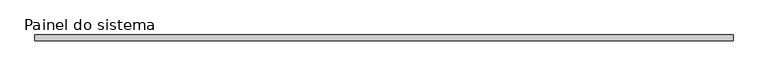
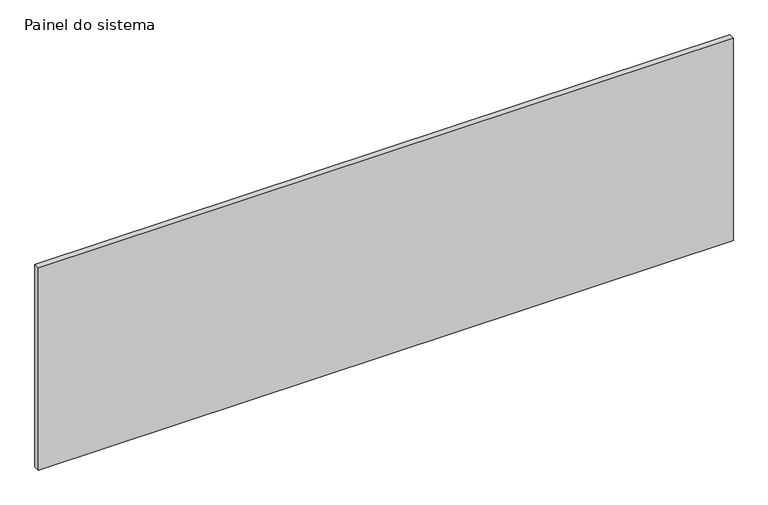
"""IFC4 building model written with IfcOpenShell, lengths in millimetres: plate geometry, Painel do sistema : Envidraçado."""

from ifc_helpers import new_model, si_unit, origin, origin_with_axes, place, context, project, spatial, polyline, outline, extrude, source, transform, mapped, element, save


def painel_do_sistema_70ab7d4e(model_context):
    return source(origin(), model_context, "Body", "SweptSolid", [
        extrude(outline(polyline([(1462.5000305, -49.5), (-1462.5000305, -49.5), (-1462.5000305, -24.5), (1462.5000305, -24.5), (1462.5000305, -49.5)])), origin_with_axes(), (0.0, 0.0, 1.0), 900.0),
    ])


if __name__ == "__main__":
    model = new_model("IFC4")
    model_context = context("Model", 3, world=origin())
    ifc_project = project(units=[si_unit("LENGTHUNIT", "METRE", prefix="MILLI")], contexts=[model_context])
    site = spatial("IfcSite", under=ifc_project)
    building = spatial("IfcBuilding", under=site)
    placement = place(None, origin())
    painel_do_sistema_shape = painel_do_sistema_70ab7d4e(model_context)
    element("IfcPlate", 1, ObjectType="Painel do sistema : Envidraçado", at=placement, inside=building, context=model_context, shape_type="MappedRepresentation", body=[
        mapped(painel_do_sistema_shape, transform((0.0, 0.0, 0.0), x_axis=(1.0, 0.0, 0.0), y_axis=(0.0, 1.0, 0.0), z_axis=(0.0, 0.0, 1.0))),
    ])
    save(model, "model.ifc")

# Revit data of these elements
# Type "Painel do sistema : Envidraçado"
#   Construction Type Id = "GSP4R"
#   Analytic Construction = "Vidraça única Pilkington 1/8 pol"
#   Visual Light Transmittance = 0.9
#   Solar Heat Gain Coefficient = 0.86
#   Heat Transfer Coefficient (U) = 6.7069 W/(m²·K)
# Element 1 (IfcPlate, "Painel do sistema : Envidraçado")
#   Materials on its faces: "Vidro"
# Materials
#   "Vidro": class "Vidro", colour RGB 0 128 192, transparency 0.9, Description = "Vidro de sílica", Cost = 0
